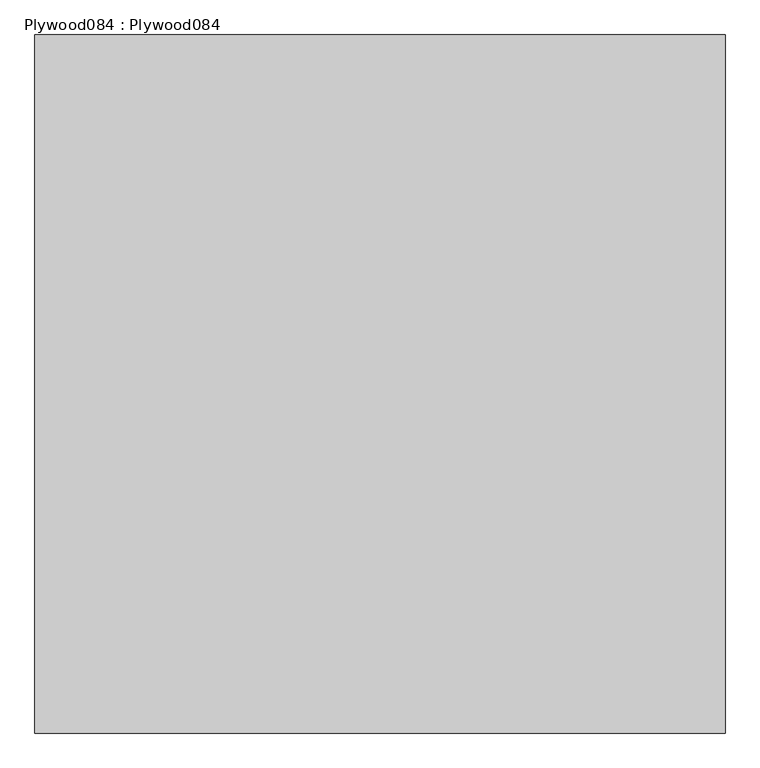
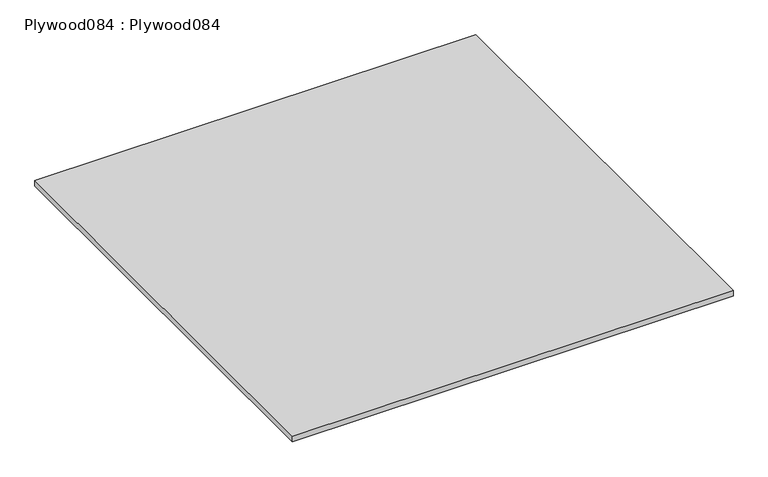
"""IFC4 building model written with IfcOpenShell, lengths in millimetres: proxy geometry, Plywood084 : Plywood084."""

from ifc_helpers import new_model, si_unit, frame, origin, place, context, project, spatial, polyline, outline, extrude, source, transform, mapped, element, save


def plywood084_plywood084_0f27dee5(model_context):
    return source(origin(), model_context, "Body", "SweptSolid", [
        extrude(outline(polyline([(-474.2526923, -1052.8906574), (-2451.1102963, -1052.8906574), (-2451.1102963, 947.1093426), (-474.2526923, 947.1093426), (-474.2526923, -1052.8906574)])), frame((0.0, 0.0, 42489.1017865), z_axis=(0.0, 0.0, 1.0), x_axis=(1.0, 0.0, 0.0)), (0.0, 0.0, 1.0), 26.0465759),
    ])


if __name__ == "__main__":
    model = new_model("IFC4")
    model_context = context("Model", 3, world=origin())
    ifc_project = project(units=[si_unit("LENGTHUNIT", "METRE", prefix="MILLI")], contexts=[model_context])
    site = spatial("IfcSite", under=ifc_project)
    building = spatial("IfcBuilding", under=site)
    placement = place(None, origin())
    plywood084_plywood084_shape = plywood084_plywood084_0f27dee5(model_context)
    element("IfcBuildingElementProxy", 1, Name="Plywood084 : Plywood084", ObjectType="Plywood084 : Plywood084", at=placement, inside=building, context=model_context, shape_type="MappedRepresentation", body=[
        mapped(plywood084_plywood084_shape, transform((0.0, 0.0, 0.0), x_axis=(1.0, 0.0, 0.0), y_axis=(0.0, 1.0, 0.0), z_axis=(0.0, 0.0, 1.0))),
    ])
    save(model, "model.ifc")

# Revit data of these elements
# Type "Plywood084 : Plywood084"
#   NameOverride = "Plywood084"
# Element 1 (IfcBuildingElementProxy, "Plywood084 : Plywood084")
#   Materials on its faces: "CDX PLYWOOD - SEE STRUCTURAL DWGS"
# Materials
#   "CDX PLYWOOD - SEE STRUCTURAL DWGS": class "Unassigned", colour RGB 177 130 114, transparency 0, Cost = 0
